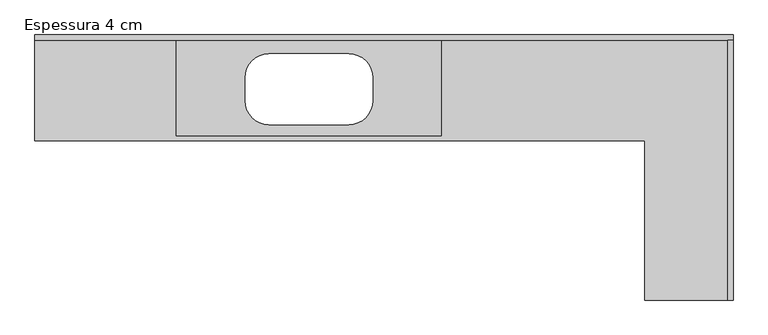
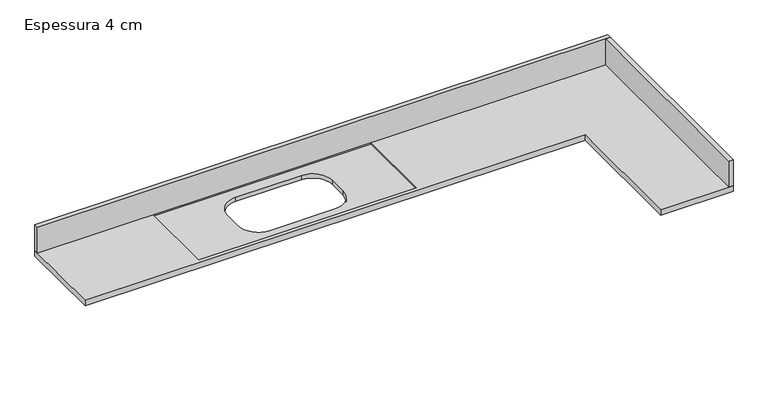
"""IFC4 building model written with IfcOpenShell, lengths in millimetres: furniture geometry, CC_BANCADA-COZINHA_EM-L_CUBA-DUPLA : Espessura 4 cm."""

from ifc_helpers import new_model, si_unit, frame, origin, place, context, project, spatial, polyline, circle_curve, outline, extrude, source, transform, mapped, element, save
from ifc_brep_helpers import plane_surface, revolved_surface, advanced_brep


def espessura_4_cm_f782d00c(model_context):
    return source(origin(), model_context, "Body", "SolidModel", [
        extrude(outline(polyline([(-30.0, -30.0), (0.0, -30.0), (0.0, -1500.0), (-30.0, -1500.0), (-30.0, -30.0)])), frame((0.0, 0.0, 900.0), z_axis=(0.0, 0.0, 1.0), x_axis=(1.0, 0.0, 0.0)), (0.0, 0.0, 1.0), 190.0),
        extrude(outline(polyline([(-3950.0, -30.0), (-3950.0, 0.0), (0.0, 0.0), (0.0, -30.0), (-3950.0, -30.0)])), frame((0.0, 0.0, 900.0), z_axis=(0.0, 0.0, 1.0), x_axis=(1.0, 0.0, 0.0)), (0.0, 0.0, 1.0), 190.0),
        advanced_brep(
        [(-500.0, -600.0, 860.0), (-3950.0, -600.0, 860.0), (-3950.0, 0.0, 860.0), (0.0, 0.0, 860.0), (0.0, -1500.0, 860.0), (-500.0, -1500.0, 860.0), (-2626.0, -107.0, 860.0), (-2761.0, -242.0, 860.0), (-2761.0, -372.0, 860.0), (-2626.0, -507.0, 860.0), (-2174.0, -507.0, 860.0), (-2039.0, -372.0, 860.0), (-2039.0, -242.0, 860.0), (-2174.0, -107.0, 860.0), (-500.0, -600.0, 900.0), (-500.0, -1500.0, 900.0), (0.0, -1500.0, 900.0), (0.0, 0.0, 900.0), (-3950.0, 0.0, 900.0), (-3950.0, -600.0, 900.0), (-1650.0, -30.0, 900.0), (-1650.0, -570.0, 900.0), (-3150.0, -570.0, 900.0), (-3150.0, -30.0, 900.0), (-2174.0, -107.0, 890.0), (-2626.0, -107.0, 890.0), (-2039.0, -242.0, 890.0), (-2039.0, -372.0, 890.0), (-2174.0, -507.0, 890.0), (-2626.0, -507.0, 890.0), (-2761.0, -372.0, 890.0), (-2761.0, -242.0, 890.0), (-1650.0, -570.0, 890.0), (-1650.0, -30.0, 890.0), (-3150.0, -30.0, 890.0), (-3150.0, -570.0, 890.0)],
        [
            (0, 1),
            (1, 2),
            (2, 3),
            (3, 4),
            (4, 5),
            (5, 0),
            (6, 7, circle_curve(frame((-2626.0, -242.0, 860.0), z_axis=(0.0, 0.0, 1.0), x_axis=(-1.0, 0.0, 0.0)), 135.0)),
            (7, 8),
            (8, 9, circle_curve(frame((-2626.0, -372.0, 860.0), z_axis=(0.0, 0.0, 1.0), x_axis=(-1.0, 0.0, 0.0)), 135.0)),
            (9, 10),
            (10, 11, circle_curve(frame((-2174.0, -372.0, 860.0), z_axis=(0.0, 0.0, 1.0), x_axis=(-1.0, 0.0, 0.0)), 135.0)),
            (11, 12),
            (12, 13, circle_curve(frame((-2174.0, -242.0, 860.0), z_axis=(0.0, 0.0, 1.0), x_axis=(-1.0, 0.0, 0.0)), 135.0)),
            (13, 6),
            (14, 15),
            (15, 16),
            (16, 17),
            (17, 18),
            (18, 19),
            (19, 14),
            (20, 21),
            (21, 22),
            (22, 23),
            (23, 20),
            (5, 15),
            (14, 0),
            (4, 16),
            (3, 17),
            (2, 18),
            (1, 19),
            (13, 24),
            (24, 25),
            (25, 6),
            (12, 26),
            (26, 24, circle_curve(frame((-2174.0, -242.0, 890.0), z_axis=(0.0, 0.0, 1.0), x_axis=(-1.0, 0.0, 0.0)), 135.0)),
            (11, 27),
            (27, 26),
            (10, 28),
            (28, 27, circle_curve(frame((-2174.0, -372.0, 890.0), z_axis=(0.0, 0.0, 1.0), x_axis=(-1.0, 0.0, 0.0)), 135.0)),
            (9, 29),
            (29, 28),
            (8, 30),
            (30, 29, circle_curve(frame((-2626.0, -372.0, 890.0), z_axis=(0.0, 0.0, 1.0), x_axis=(-1.0, 0.0, 0.0)), 135.0)),
            (7, 31),
            (31, 30),
            (25, 31, circle_curve(frame((-2626.0, -242.0, 890.0), z_axis=(0.0, 0.0, 1.0), x_axis=(-1.0, 0.0, 0.0)), 135.0)),
            (32, 33),
            (33, 34),
            (34, 35),
            (35, 32),
            (32, 21),
            (20, 33),
            (23, 34),
            (22, 35),
        ],
        [
            plane_surface(frame((-500.0, -600.0, 860.0), z_axis=(0.0, 0.0, -1.0), x_axis=(0.0, 1.0, 0.0))),
            plane_surface(frame((-500.0, -600.0, 900.0), z_axis=(0.0, 0.0, 1.0), x_axis=(0.0, -1.0, 0.0))),
            plane_surface(frame((-500.0, -600.0, 900.0), z_axis=(-1.0, 0.0, 0.0), x_axis=(0.0, 0.0, -1.0))),
            plane_surface(frame((-500.0, -1500.0, 900.0), z_axis=(0.0, -1.0, 0.0), x_axis=(0.0, 0.0, -1.0))),
            plane_surface(frame((0.0, -1500.0, 900.0), z_axis=(1.0, 0.0, 0.0), x_axis=(0.0, 0.0, -1.0))),
            plane_surface(frame((0.0, 0.0, 900.0), z_axis=(0.0, 1.0, 0.0), x_axis=(0.0, 0.0, -1.0))),
            plane_surface(frame((-3950.0, 0.0, 900.0), z_axis=(-1.0, 0.0, 0.0), x_axis=(0.0, 0.0, -1.0))),
            plane_surface(frame((-3950.0, -600.0, 900.0), z_axis=(0.0, -1.0, 0.0), x_axis=(0.0, 0.0, -1.0))),
            plane_surface(frame((-2626.0, -107.0, 900.0), z_axis=(0.0, -1.0, 0.0), x_axis=(0.0, 0.0, -1.0))),
            revolved_surface(polyline([(-2309.0, -242.0, 860.0), (-2309.0, -242.0, 890.0)]), (-2174.0, -242.0, 890.0), (0.0, 0.0, -1.0)),
            plane_surface(frame((-2039.0, -242.0, 900.0), z_axis=(-1.0, 0.0, 0.0), x_axis=(0.0, 0.0, -1.0))),
            revolved_surface(polyline([(-2309.0, -372.0, 860.0), (-2309.0, -372.0, 890.0)]), (-2174.0, -372.0, 890.0), (0.0, 0.0, -1.0)),
            plane_surface(frame((-2174.0, -507.0, 900.0), z_axis=(0.0, 1.0, 0.0), x_axis=(0.0, 0.0, -1.0))),
            revolved_surface(polyline([(-2761.0, -372.0, 860.0), (-2761.0, -372.0, 890.0)]), (-2626.0, -372.0, 890.0), (0.0, 0.0, -1.0)),
            plane_surface(frame((-2761.0, -372.0, 900.0), z_axis=(1.0, 0.0, 0.0), x_axis=(0.0, 0.0, -1.0))),
            revolved_surface(polyline([(-2761.0, -242.0, 860.0), (-2761.0, -242.0, 890.0)]), (-2626.0, -242.0, 890.0), (0.0, 0.0, -1.0)),
            plane_surface(frame((-1650.0, -30.0, 890.0), z_axis=(0.0, 0.0, 1.0), x_axis=(0.0, -1.0, 0.0))),
            plane_surface(frame((-1650.0, -570.0, 940.0), z_axis=(-1.0, 0.0, 0.0), x_axis=(0.0, 0.0, -1.0))),
            plane_surface(frame((-1650.0, -30.0, 940.0), z_axis=(0.0, -1.0, 0.0), x_axis=(0.0, 0.0, -1.0))),
            plane_surface(frame((-3150.0, -30.0, 940.0), z_axis=(1.0, 0.0, 0.0), x_axis=(0.0, 0.0, -1.0))),
            plane_surface(frame((-3150.0, -570.0, 940.0), z_axis=(0.0, 1.0, 0.0), x_axis=(0.0, 0.0, -1.0))),
        ],
        [
            (0, [[1, 2, 3, 4, 5, 6], [7, 8, 9, 10, 11, 12, 13, 14]]),
            (1, [[15, 16, 17, 18, 19, 20], [21, 22, 23, 24]]),
            (2, [[-6, 25, -15, 26]]),
            (3, [[-5, 27, -16, -25]]),
            (4, [[-4, 28, -17, -27]]),
            (5, [[-3, 29, -18, -28]]),
            (6, [[-2, 30, -19, -29]]),
            (7, [[-1, -26, -20, -30]]),
            (8, [[-14, 31, 32, 33]]),
            (9, [[-13, 34, 35, -31]]),
            (10, [[-12, 36, 37, -34]]),
            (11, [[-11, 38, 39, -36]]),
            (12, [[-10, 40, 41, -38]]),
            (13, [[-9, 42, 43, -40]]),
            (14, [[-8, 44, 45, -42]]),
            (15, [[-7, -33, 46, -44]]),
            (16, [[47, 48, 49, 50], [-32, -35, -37, -39, -41, -43, -45, -46]]),
            (17, [[-47, 51, -21, 52]]),
            (18, [[-48, -52, -24, 53]]),
            (19, [[-49, -53, -23, 54]]),
            (20, [[-50, -54, -22, -51]]),
        ],
    ),
    ])


if __name__ == "__main__":
    model = new_model("IFC4")
    model_context = context("Model", 3, world=origin())
    ifc_project = project(units=[si_unit("LENGTHUNIT", "METRE", prefix="MILLI")], contexts=[model_context])
    site = spatial("IfcSite", under=ifc_project)
    building = spatial("IfcBuilding", under=site)
    placement = place(None, origin())
    espessura_4_cm_shape = espessura_4_cm_f782d00c(model_context)
    element("IfcFurniture", 1, ObjectType="CC_BANCADA-COZINHA_EM-L_CUBA-DUPLA : Espessura 4 cm", at=placement, inside=building, context=model_context, shape_type="MappedRepresentation", body=[
        mapped(espessura_4_cm_shape, transform((0.0, 0.0, 0.0), x_axis=(1.0, 0.0, 0.0), y_axis=(0.0, 1.0, 0.0), z_axis=(0.0, 0.0, 1.0))),
    ])
    save(model, "model.ifc")

# Revit data of these elements
# Type "CC_BANCADA-COZINHA_EM-L_CUBA-DUPLA : Espessura 4 cm"
#   Uso HS [instance default] = ""
#   Offset esq área molhada [instance default] = 0.80 m
#   Largura área molhada [instance default] = 1.50 m
#   Largura principal [instance default] = 0.60 m
#   Largura da extensão [instance default] = 0.50 m
#   Espessura total da bancada [instance default] = 0.04 m
#   Espessura do frontão [instance default] = 0.03 m
#   Dist. cuba - borda [instance default] = 0.07 m
#   Compr. total principal [instance default] = 3.95 m
#   Compr. principal [instance default] = 3.45 m
#   Compr. total extensão [instance default] = 1.50 m
#   Compr. extensão [instance default] = 0.90 m
#   Altura do rebaixo da área molhada [instance default] = 0.01 m
#   Altura do frontão [instance default] = 0.20 m
#   Altura da bancada [instance default] = 0.90 m
#   Frontão fundos principal [instance default] = yes
#   Frontão fundos extensão [instance default] = yes
#   Frontão esquerdo principal [instance default] = yes
#   Frontão direito extensão [instance default] = yes
#   Material da bancada [instance default] = none
# Element 1 (IfcFurniture, "CC_BANCADA-COZINHA_EM-L_CUBA-DUPLA : Espessura 4 cm")
#   Uso HS = "COZINHA"
#   Frontão esquerdo principal = no
#   Frontão direito extensão = no
#   Material da bancada = .GRANITO_BRANCO_ITAUNAS
#   Materials on its faces: ".GRANITO_BRANCO_ITAUNAS"
# Materials
#   ".GRANITO_BRANCO_ITAUNAS": class ".CC_PEDRA REVEST.", colour RGB 202 195 174, transparency 0, Description = "Revestimento em granito", Cost = 0
